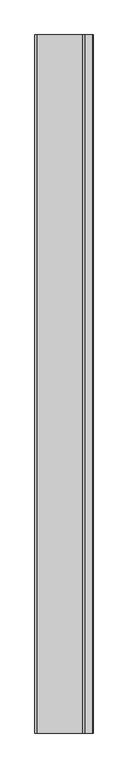
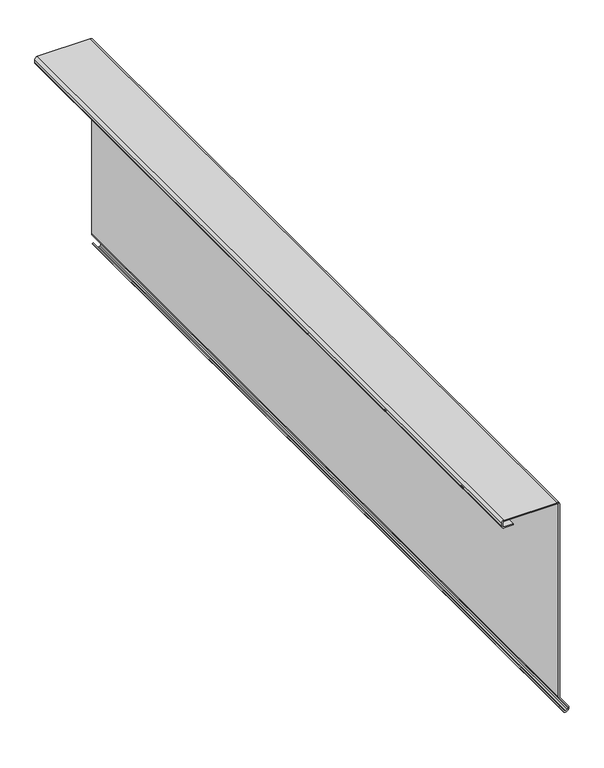
"""IFC4 building model written with IfcOpenShell, lengths in millimetres: proxy geometry, Flashing024 12494 : Flashing024 12494."""

from ifc_helpers import new_model, si_unit, point, frame, frame_2d, origin, place, context, project, spatial, polyline, circle_curve, trimmed, segment, composite_curve, outline, extrude, source, transform, mapped, element, save


def generic_models_84a2b06a(model_context):
    return source(origin(), model_context, "Body", "SweptSolid", [
        extrude(outline(composite_curve([segment(trimmed(circle_curve(frame_2d((41300.7116849, 6188.9556944)), 6.35), [point((41297.0425395, 6183.7730434))], [point((41295.2345891, 6192.1687804))], False, "CARTESIAN"), True, "CONTINUOUS"), segment(polyline([(41295.2345891, 6192.1687804), (41296.9758154, 6195.1369125)]), True, "CONTINUOUS"), segment(trimmed(circle_curve(frame_2d((41302.4529113, 6191.9238265)), 6.35), [point((41296.9758154, 6195.1369125))], [point((41306.0703854, 6197.1426751))], False, "CARTESIAN"), True, "CONTINUOUS"), segment(polyline([(41306.0703854, 6197.1426751), (41336.0634258, 6176.3528311)]), True, "CONTINUOUS"), segment(trimmed(circle_curve(frame_2d((41339.6809, 6181.5716797)), 6.35), [point((41336.0634258, 6176.3528311))], [point((41339.6809, 6175.2216797))], True, "CARTESIAN"), True, "CONTINUOUS"), segment(polyline([(41339.6809, 6175.2216797), (41842.9189039, 6175.2216797)]), True, "CONTINUOUS"), segment(trimmed(circle_curve(frame_2d((41842.9189039, 6168.8716797)), 6.35), [point((41842.9189039, 6175.2216797))], [point((41849.2689039, 6168.8716797))], False, "CARTESIAN"), True, "CONTINUOUS"), segment(polyline([(41849.2689039, 6168.8716797), (41849.2689039, 6038.1540605)]), True, "CONTINUOUS"), segment(trimmed(circle_curve(frame_2d((41842.9189039, 6038.1540605)), 6.35), [point((41849.2689039, 6038.1540605))], [point((41842.9189039, 6031.8040605))], False, "CARTESIAN"), True, "CONTINUOUS"), segment(polyline([(41842.9189039, 6031.8040605), (41835.0524976, 6031.8040605)]), True, "CONTINUOUS"), segment(trimmed(circle_curve(frame_2d((41835.0524976, 6038.1540605)), 6.35), [point((41835.0524976, 6031.8040605))], [point((41828.7024976, 6038.1540605))], False, "CARTESIAN"), True, "CONTINUOUS"), segment(polyline([(41828.7024976, 6038.1540605), (41828.7024976, 6060.1805253), (41831.7024976, 6060.1805253), (41831.7024976, 6038.1540605)]), True, "CONTINUOUS"), segment(trimmed(circle_curve(frame_2d((41835.0524976, 6038.1540605)), 3.35), [point((41831.7024976, 6038.1540605))], [point((41835.0524976, 6034.8040605))], True, "CARTESIAN"), True, "CONTINUOUS"), segment(polyline([(41835.0524976, 6034.8040605), (41842.9189039, 6034.8040605)]), True, "CONTINUOUS"), segment(trimmed(circle_curve(frame_2d((41842.9189039, 6038.1540605)), 3.35), [point((41842.9189039, 6034.8040605))], [point((41846.2689039, 6038.1540605))], True, "CARTESIAN"), True, "CONTINUOUS"), segment(polyline([(41846.2689039, 6038.1540605), (41846.2689039, 6168.8716797)]), True, "CONTINUOUS"), segment(trimmed(circle_curve(frame_2d((41842.9189039, 6168.8716797)), 3.35), [point((41846.2689039, 6168.8716797))], [point((41842.9189039, 6172.2216797))], True, "CARTESIAN"), True, "CONTINUOUS"), segment(polyline([(41842.9189039, 6172.2216797), (41339.6809, 6172.2216797)]), True, "CONTINUOUS"), segment(trimmed(circle_curve(frame_2d((41339.6809, 6181.5716797)), 9.35), [point((41339.6809, 6172.2216797))], [point((41334.3543829, 6173.8872333))], False, "CARTESIAN"), True, "CONTINUOUS"), segment(polyline([(41334.3543829, 6173.8872333), (41304.3613425, 6194.6770774)]), True, "CONTINUOUS"), segment(trimmed(circle_curve(frame_2d((41302.4529113, 6191.9238265)), 3.35), [point((41304.3613425, 6194.6770774))], [point((41299.5634198, 6193.6189191))], True, "CARTESIAN"), True, "CONTINUOUS"), segment(polyline([(41299.5634198, 6193.6189191), (41297.8221934, 6190.650787)]), True, "CONTINUOUS"), segment(trimmed(circle_curve(frame_2d((41300.7116849, 6188.9556944)), 3.35), [point((41297.8221934, 6190.650787))], [point((41298.7759941, 6186.2215399))], True, "CARTESIAN"), True, "CONTINUOUS"), segment(polyline([(41298.7759941, 6186.2215399), (41313.5223857, 6175.7815827), (41311.7889312, 6173.3330862), (41297.0425395, 6183.7730434)]), True, "CONTINUOUS")], self_intersect=False)), frame((0.0, 2217.3609988, 0.0), z_axis=(0.0, 1.0, 0.0), x_axis=(0.0, 0.0, 1.0)), (0.0, 0.0, 1.0), 2000.0),
    ])


if __name__ == "__main__":
    model = new_model("IFC4")
    model_context = context("Model", 3, world=origin())
    ifc_project = project(units=[si_unit("LENGTHUNIT", "METRE", prefix="MILLI")], contexts=[model_context])
    site = spatial("IfcSite", under=ifc_project)
    building = spatial("IfcBuilding", under=site)
    placement = place(None, origin())
    generic_models_shape = generic_models_84a2b06a(model_context)
    element("IfcBuildingElementProxy", 1, Name="Flashing024 12494 : Flashing024 12494", ObjectType="Flashing024 12494 : Flashing024 12494", at=placement, inside=building, context=model_context, shape_type="MappedRepresentation", body=[
        mapped(generic_models_shape, transform((0.0, 0.0, 0.0), x_axis=(1.0, 0.0, 0.0), y_axis=(0.0, 1.0, 0.0), z_axis=(0.0, 0.0, 1.0))),
    ])
    save(model, "model.ifc")

# Revit data of these elements
# Type "Flashing024 12494 : Flashing024 12494"
#   NameOverride = "Flashing024"
# Element 1 (IfcBuildingElementProxy, "Flashing024 12494 : Flashing024 12494")
#   Materials on its faces: "HIGH EAVE FLASHING"
# Materials
#   "HIGH EAVE FLASHING": class "Unassigned", colour RGB 128 128 128, transparency 0
